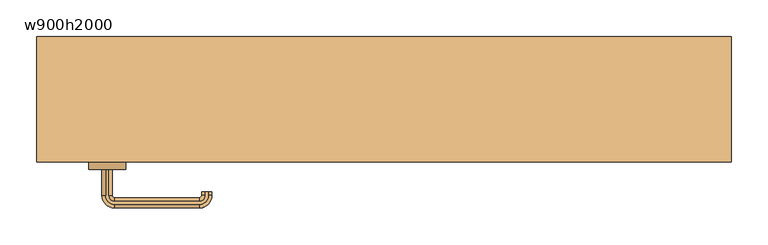
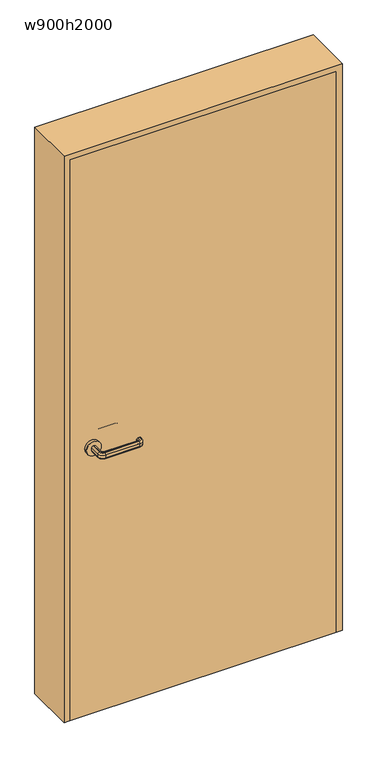
"""IFC4 building model written with IfcOpenShell, lengths in millimetres: door geometry, 片開き : w900h2000."""

from ifc_helpers import new_model, si_unit, point, frame, frame_2d, origin, origin_with_axes, place, context, project, spatial, polyline, circle_curve, ellipse_curve, trimmed, segment, composite_curve, outline, extrude, source, transform, mapped, element, save
from ifc_brep_helpers import plane_surface, cylinder_surface, revolved_surface, advanced_brep


def w900h2000_c063673d(model_context):
    return source(origin(), model_context, "Body", "SolidModel", [
        advanced_brep(
        [(-377.0, -95.0, 960.0), (-373.0, -95.0, 960.0), (-368.0, -95.0, 955.0), (-368.0, -95.0, 945.0477623), (-373.0, -95.0, 940.0477623), (-377.0, -95.0, 940.0477623), (-382.0, -95.0, 945.0477623), (-382.0, -95.0, 955.0), (-382.0, -130.0, 955.0), (-377.0, -130.0, 960.0), (-382.0, -130.0, 945.0477623), (-377.0, -130.0, 940.0477623), (-373.0, -130.0, 940.0477623), (-365.0, -138.0, 940.0477623), (-250.0, -138.0, 940.0477623), (-242.0, -130.0, 940.0477623), (-242.0, -125.0, 940.0477623), (-238.0, -125.0, 940.0477623), (-238.0, -130.0, 940.0477623), (-250.0, -142.0, 940.0477623), (-365.0, -142.0, 940.0477623), (-368.0, -130.0, 945.0477623), (-368.0, -130.0, 955.0), (-373.0, -130.0, 960.0), (-365.0, -142.0, 960.0), (-250.0, -142.0, 960.0), (-238.0, -130.0, 960.0), (-238.0, -125.0, 960.0), (-242.0, -125.0, 960.0), (-242.0, -130.0, 960.0), (-250.0, -138.0, 960.0), (-365.0, -138.0, 960.0), (-365.0, -147.0, 955.0), (-365.0, -147.0, 945.0477623), (-365.0, -133.0, 945.0477623), (-365.0, -133.0, 955.0), (-250.0, -147.0, 955.0), (-250.0, -147.0, 945.0477623), (-250.0, -133.0, 945.0477623), (-250.0, -133.0, 955.0), (-233.0, -130.0, 955.0), (-233.0, -130.0, 945.0477623), (-247.0, -130.0, 945.0477623), (-247.0, -130.0, 955.0), (-233.0, -125.0, 955.0), (-233.0, -125.0, 945.0477623), (-247.0, -125.0, 945.0477623), (-247.0, -125.0, 955.0)],
        [
            (0, 1),
            (1, 2, circle_curve(frame((-373.0, -95.0, 955.0), z_axis=(0.0, 1.0, 0.0), x_axis=(-1.0, 0.0, 0.0)), 5.0)),
            (2, 3),
            (3, 4, circle_curve(frame((-373.0, -95.0, 945.0477623), z_axis=(0.0, 1.0, 0.0), x_axis=(-1.0, 0.0, 0.0)), 5.0)),
            (4, 5),
            (5, 6, circle_curve(frame((-377.0, -95.0, 945.0477623), z_axis=(0.0, 1.0, 0.0), x_axis=(-1.0, 0.0, 0.0)), 5.0)),
            (6, 7),
            (7, 0, circle_curve(frame((-377.0, -95.0, 955.0), z_axis=(0.0, 1.0, 0.0), x_axis=(-1.0, 0.0, 0.0)), 5.0)),
            (7, 8),
            (8, 9, circle_curve(frame((-377.0, -130.0, 955.0), z_axis=(0.0, 1.0, 0.0), x_axis=(-1.0, 0.0, 0.0)), 5.0)),
            (9, 0),
            (6, 10),
            (10, 8),
            (5, 11),
            (11, 10, circle_curve(frame((-377.0, -130.0, 945.0477623), z_axis=(0.0, 1.0, 0.0), x_axis=(-1.0, 0.0, 0.0)), 5.0)),
            (4, 12),
            (12, 13, circle_curve(frame((-365.0, -130.0, 940.0477623), z_axis=(0.0, 0.0, 1.0), x_axis=(-1.0, 0.0, 0.0)), 8.0)),
            (13, 14),
            (14, 15, circle_curve(frame((-250.0, -130.0, 940.0477623), z_axis=(0.0, 0.0, 1.0), x_axis=(0.0, -1.0, 0.0)), 8.0)),
            (15, 16),
            (16, 17),
            (17, 18),
            (18, 19, circle_curve(frame((-250.0, -130.0, 940.0477623), z_axis=(0.0, 0.0, -1.0), x_axis=(0.0, -1.0, 0.0)), 12.0)),
            (19, 20),
            (20, 11, circle_curve(frame((-365.0, -130.0, 940.0477623), z_axis=(0.0, 0.0, -1.0), x_axis=(-1.0, 0.0, 0.0)), 12.0)),
            (3, 21),
            (21, 12, circle_curve(frame((-373.0, -130.0, 945.0477623), z_axis=(0.0, 1.0, 0.0), x_axis=(-1.0, 0.0, 0.0)), 5.0)),
            (2, 22),
            (22, 21),
            (1, 23),
            (23, 22, circle_curve(frame((-373.0, -130.0, 955.0), z_axis=(0.0, 1.0, 0.0), x_axis=(-1.0, 0.0, 0.0)), 5.0)),
            (9, 24, circle_curve(frame((-365.0, -130.0, 960.0), z_axis=(0.0, 0.0, 1.0), x_axis=(-1.0, 0.0, 0.0)), 12.0)),
            (24, 25),
            (25, 26, circle_curve(frame((-250.0, -130.0, 960.0), z_axis=(0.0, 0.0, 1.0), x_axis=(0.0, -1.0, 0.0)), 12.0)),
            (26, 27),
            (27, 28),
            (28, 29),
            (29, 30, circle_curve(frame((-250.0, -130.0, 960.0), z_axis=(0.0, 0.0, -1.0), x_axis=(0.0, -1.0, 0.0)), 8.0)),
            (30, 31),
            (31, 23, circle_curve(frame((-365.0, -130.0, 960.0), z_axis=(0.0, 0.0, -1.0), x_axis=(-1.0, 0.0, 0.0)), 8.0)),
            (32, 24, circle_curve(frame((-365.0, -142.0, 955.0), z_axis=(-1.0, 0.0, 0.0), x_axis=(0.0, -1.0, 0.0)), 5.0)),
            (8, 32, circle_curve(frame((-365.0, -130.0, 955.0), z_axis=(0.0, 0.0, 1.0), x_axis=(-1.0, 0.0, 0.0)), 17.0)),
            (33, 32),
            (10, 33, circle_curve(frame((-365.0, -130.0, 945.0477623), z_axis=(0.0, 0.0, 1.0), x_axis=(-1.0, 0.0, 0.0)), 17.0)),
            (20, 33, circle_curve(frame((-365.0, -142.0, 945.0477623), z_axis=(-1.0, 0.0, 0.0), x_axis=(0.0, -1.0, 0.0)), 5.0)),
            (34, 13, circle_curve(frame((-365.0, -138.0, 945.0477623), z_axis=(-1.0, 0.0, 0.0), x_axis=(0.0, -1.0, 0.0)), 5.0)),
            (21, 34, circle_curve(frame((-365.0, -130.0, 945.0477623), z_axis=(0.0, 0.0, 1.0), x_axis=(-1.0, 0.0, 0.0)), 3.0)),
            (35, 34),
            (22, 35, circle_curve(frame((-365.0, -130.0, 955.0), z_axis=(0.0, 0.0, 1.0), x_axis=(-1.0, 0.0, 0.0)), 3.0)),
            (31, 35, circle_curve(frame((-365.0, -138.0, 955.0), z_axis=(-1.0, 0.0, 0.0), x_axis=(0.0, -1.0, 0.0)), 5.0)),
            (32, 36),
            (36, 25, circle_curve(frame((-250.0, -142.0, 955.0), z_axis=(-1.0, 0.0, 0.0), x_axis=(0.0, -1.0, 0.0)), 5.0)),
            (33, 37),
            (37, 36),
            (19, 37, circle_curve(frame((-250.0, -142.0, 945.0477623), z_axis=(-1.0, 0.0, 0.0), x_axis=(0.0, -1.0, 0.0)), 5.0)),
            (34, 38),
            (38, 14, circle_curve(frame((-250.0, -138.0, 945.0477623), z_axis=(-1.0, 0.0, 0.0), x_axis=(0.0, -1.0, 0.0)), 5.0)),
            (35, 39),
            (39, 38),
            (30, 39, circle_curve(frame((-250.0, -138.0, 955.0), z_axis=(-1.0, 0.0, 0.0), x_axis=(0.0, -1.0, 0.0)), 5.0)),
            (40, 26, circle_curve(frame((-238.0, -130.0, 955.0), z_axis=(0.0, -1.0, 0.0), x_axis=(1.0, 0.0, 0.0)), 5.0)),
            (36, 40, circle_curve(frame((-250.0, -130.0, 955.0), z_axis=(0.0, 0.0, 1.0), x_axis=(0.0, -1.0, 0.0)), 17.0)),
            (41, 40),
            (37, 41, circle_curve(frame((-250.0, -130.0, 945.0477623), z_axis=(0.0, 0.0, 1.0), x_axis=(0.0, -1.0, 0.0)), 17.0)),
            (18, 41, circle_curve(frame((-238.0, -130.0, 945.0477623), z_axis=(0.0, -1.0, 0.0), x_axis=(1.0, 0.0, 0.0)), 5.0)),
            (42, 15, circle_curve(frame((-242.0, -130.0, 945.0477623), z_axis=(0.0, -1.0, 0.0), x_axis=(1.0, 0.0, 0.0)), 5.0)),
            (38, 42, circle_curve(frame((-250.0, -130.0, 945.0477623), z_axis=(0.0, 0.0, 1.0), x_axis=(0.0, -1.0, 0.0)), 3.0)),
            (43, 42),
            (39, 43, circle_curve(frame((-250.0, -130.0, 955.0), z_axis=(0.0, 0.0, 1.0), x_axis=(0.0, -1.0, 0.0)), 3.0)),
            (29, 43, circle_curve(frame((-242.0, -130.0, 955.0), z_axis=(0.0, -1.0, 0.0), x_axis=(1.0, 0.0, 0.0)), 5.0)),
            (27, 44, circle_curve(frame((-238.0, -125.0, 955.0), z_axis=(0.0, 1.0, 0.0), x_axis=(1.0, 0.0, 0.0)), 5.0)),
            (44, 45),
            (45, 17, circle_curve(frame((-238.0, -125.0, 945.0477623), z_axis=(0.0, 1.0, 0.0), x_axis=(1.0, 0.0, 0.0)), 5.0)),
            (16, 46, circle_curve(frame((-242.0, -125.0, 945.0477623), z_axis=(0.0, 1.0, 0.0), x_axis=(1.0, 0.0, 0.0)), 5.0)),
            (46, 47),
            (47, 28, circle_curve(frame((-242.0, -125.0, 955.0), z_axis=(0.0, 1.0, 0.0), x_axis=(1.0, 0.0, 0.0)), 5.0)),
            (40, 44),
            (41, 45),
            (42, 46),
            (43, 47),
        ],
        [
            plane_surface(frame((-385.198039, -95.0, 950.0), z_axis=(0.0, 1.0, 0.0), x_axis=(0.0, 0.0, 1.0))),
            cylinder_surface(frame((-377.0, -95.0, 955.0), z_axis=(0.0, 1.0, 0.0), x_axis=(-1.0, 0.0, 0.0)), 5.0),
            plane_surface(frame((-382.0, -95.0, 955.0), z_axis=(-1.0, 0.0, 0.0), x_axis=(0.0, -1.0, 0.0))),
            cylinder_surface(frame((-377.0, -95.0, 945.0477623), z_axis=(0.0, 1.0, 0.0), x_axis=(-1.0, 0.0, 0.0)), 5.0),
            plane_surface(frame((-377.0, -95.0, 940.0477623), z_axis=(0.0, 0.0, -1.0), x_axis=(0.0, -1.0, 0.0))),
            cylinder_surface(frame((-373.0, -95.0, 945.0477623), z_axis=(0.0, 1.0, 0.0), x_axis=(-1.0, 0.0, 0.0)), 5.0),
            plane_surface(frame((-368.0, -95.0, 945.0477623), z_axis=(1.0, 0.0, 0.0), x_axis=(0.0, -1.0, 0.0))),
            cylinder_surface(frame((-373.0, -95.0, 955.0), z_axis=(0.0, 1.0, 0.0), x_axis=(-1.0, 0.0, 0.0)), 5.0),
            plane_surface(frame((-373.0, -95.0, 960.0), z_axis=(0.0, 0.0, 1.0), x_axis=(0.0, -1.0, 0.0))),
            revolved_surface(trimmed(ellipse_curve(frame((-377.0, -130.0, 955.0), z_axis=(0.0, -1.0, 0.0), x_axis=(-1.0, 0.0, 0.0)), 5.0, 5.0), [point((-377.0, -130.0, 960.0))], [point((-382.0, -130.0, 955.0))], True, "CARTESIAN"), (-365.0, -130.0, 950.0), (0.0, 0.0, -1.0)),
            cylinder_surface(frame((-365.0, -130.0, 950.0), z_axis=(0.0, 0.0, -1.0), x_axis=(-1.0, 0.0, 0.0)), 17.0),
            revolved_surface(trimmed(ellipse_curve(frame((-377.0, -130.0, 945.0477623), z_axis=(0.0, -1.0, 0.0), x_axis=(-1.0, 0.0, 0.0)), 5.0, 5.0), [point((-382.0, -130.0, 945.0477623))], [point((-377.0, -130.0, 940.0477623))], True, "CARTESIAN"), (-365.0, -130.0, 950.0), (0.0, 0.0, -1.0)),
            revolved_surface(trimmed(ellipse_curve(frame((-373.0, -130.0, 945.0477623), z_axis=(0.0, -1.0, 0.0), x_axis=(-1.0, 0.0, 0.0)), 5.0, 5.0), [point((-373.0, -130.0, 940.0477623))], [point((-368.0, -130.0, 945.0477623))], True, "CARTESIAN"), (-365.0, -130.0, 950.0), (0.0, 0.0, -1.0)),
            revolved_surface(polyline([(-368.0, -130.0, 945.0477623), (-368.0, -130.0, 955.0)]), (-365.0, -130.0, 950.0), (0.0, 0.0, -1.0)),
            revolved_surface(trimmed(ellipse_curve(frame((-373.0, -130.0, 955.0), z_axis=(0.0, -1.0, 0.0), x_axis=(-1.0, 0.0, 0.0)), 5.0, 5.0), [point((-368.0, -130.0, 955.0))], [point((-373.0, -130.0, 960.0))], True, "CARTESIAN"), (-365.0, -130.0, 950.0), (0.0, 0.0, -1.0)),
            cylinder_surface(frame((-365.0, -142.0, 955.0), z_axis=(-1.0, 0.0, 0.0), x_axis=(0.0, -1.0, 0.0)), 5.0),
            plane_surface(frame((-365.0, -147.0, 955.0), z_axis=(0.0, -1.0, 0.0), x_axis=(1.0, 0.0, 0.0))),
            cylinder_surface(frame((-365.0, -142.0, 945.0477623), z_axis=(-1.0, 0.0, 0.0), x_axis=(0.0, -1.0, 0.0)), 5.0),
            cylinder_surface(frame((-365.0, -138.0, 945.0477623), z_axis=(-1.0, 0.0, 0.0), x_axis=(0.0, -1.0, 0.0)), 5.0),
            plane_surface(frame((-365.0, -133.0, 945.0477623), z_axis=(0.0, 1.0, 0.0), x_axis=(1.0, 0.0, 0.0))),
            cylinder_surface(frame((-365.0, -138.0, 955.0), z_axis=(-1.0, 0.0, 0.0), x_axis=(0.0, -1.0, 0.0)), 5.0),
            revolved_surface(trimmed(ellipse_curve(frame((-250.0, -142.0, 955.0), z_axis=(1.0, 0.0, 0.0), x_axis=(0.0, -1.0, 0.0)), 5.0, 5.0), [point((-250.0, -142.0, 960.0))], [point((-250.0, -147.0, 955.0))], True, "CARTESIAN"), (-250.0, -130.0, 950.0), (0.0, 0.0, -1.0)),
            cylinder_surface(frame((-250.0, -130.0, 950.0), z_axis=(0.0, 0.0, -1.0), x_axis=(0.0, -1.0, 0.0)), 17.0),
            revolved_surface(trimmed(ellipse_curve(frame((-250.0, -142.0, 945.0477623), z_axis=(1.0, 0.0, 0.0), x_axis=(0.0, -1.0, 0.0)), 5.0, 5.0), [point((-250.0, -147.0, 945.0477623))], [point((-250.0, -142.0, 940.0477623))], True, "CARTESIAN"), (-250.0, -130.0, 950.0), (0.0, 0.0, -1.0)),
            revolved_surface(trimmed(ellipse_curve(frame((-250.0, -138.0, 945.0477623), z_axis=(1.0, 0.0, 0.0), x_axis=(0.0, -1.0, 0.0)), 5.0, 5.0), [point((-250.0, -138.0, 940.0477623))], [point((-250.0, -133.0, 945.0477623))], True, "CARTESIAN"), (-250.0, -130.0, 950.0), (0.0, 0.0, -1.0)),
            revolved_surface(polyline([(-250.0, -133.0, 945.0477623), (-250.0, -133.0, 955.0)]), (-250.0, -130.0, 950.0), (0.0, 0.0, -1.0)),
            revolved_surface(trimmed(ellipse_curve(frame((-250.0, -138.0, 955.0), z_axis=(1.0, 0.0, 0.0), x_axis=(0.0, -1.0, 0.0)), 5.0, 5.0), [point((-250.0, -133.0, 955.0))], [point((-250.0, -138.0, 960.0))], True, "CARTESIAN"), (-250.0, -130.0, 950.0), (0.0, 0.0, -1.0)),
            plane_surface(frame((-250.198039, -125.0, 950.0), z_axis=(0.0, 1.0, 0.0), x_axis=(0.0, 0.0, -1.0))),
            cylinder_surface(frame((-238.0, -130.0, 955.0), z_axis=(0.0, -1.0, 0.0), x_axis=(1.0, 0.0, 0.0)), 5.0),
            plane_surface(frame((-233.0, -130.0, 955.0), z_axis=(1.0, 0.0, 0.0), x_axis=(0.0, 1.0, 0.0))),
            cylinder_surface(frame((-238.0, -130.0, 945.0477623), z_axis=(0.0, -1.0, 0.0), x_axis=(1.0, 0.0, 0.0)), 5.0),
            cylinder_surface(frame((-242.0, -130.0, 945.0477623), z_axis=(0.0, -1.0, 0.0), x_axis=(1.0, 0.0, 0.0)), 5.0),
            plane_surface(frame((-247.0, -130.0, 945.0477623), z_axis=(-1.0, 0.0, 0.0), x_axis=(0.0, 1.0, 0.0))),
            cylinder_surface(frame((-242.0, -130.0, 955.0), z_axis=(0.0, -1.0, 0.0), x_axis=(1.0, 0.0, 0.0)), 5.0),
        ],
        [
            (0, [[1, 2, 3, 4, 5, 6, 7, 8]]),
            (1, [[9, 10, 11, -8]]),
            (2, [[12, 13, -9, -7]]),
            (3, [[14, 15, -12, -6]]),
            (4, [[16, 17, 18, 19, 20, 21, 22, 23, 24, 25, -14, -5]]),
            (5, [[26, 27, -16, -4]]),
            (6, [[28, 29, -26, -3]]),
            (7, [[30, 31, -28, -2]]),
            (8, [[-11, 32, 33, 34, 35, 36, 37, 38, 39, 40, -30, -1]]),
            (9, [[41, -32, -10, 42]]),
            (10, [[43, -42, -13, 44]]),
            (11, [[45, -44, -15, -25]]),
            (12, [[46, -17, -27, 47]]),
            (13, [[48, -47, -29, 49]]),
            (14, [[50, -49, -31, -40]]),
            (15, [[51, 52, -33, -41]]),
            (16, [[53, 54, -51, -43]]),
            (17, [[-24, 55, -53, -45]]),
            (18, [[56, 57, -18, -46]]),
            (19, [[58, 59, -56, -48]]),
            (20, [[-39, 60, -58, -50]]),
            (21, [[61, -34, -52, 62]]),
            (22, [[63, -62, -54, 64]]),
            (23, [[65, -64, -55, -23]]),
            (24, [[66, -19, -57, 67]]),
            (25, [[68, -67, -59, 69]]),
            (26, [[70, -69, -60, -38]]),
            (27, [[71, 72, 73, -21, 74, 75, 76, -36]]),
            (28, [[77, -71, -35, -61]]),
            (29, [[78, -72, -77, -63]]),
            (30, [[-22, -73, -78, -65]]),
            (31, [[79, -74, -20, -66]]),
            (32, [[80, -75, -79, -68]]),
            (33, [[-37, -76, -80, -70]]),
        ],
    ),
        advanced_brep(
        [(-373.0, -45.0, 940.0), (-368.0, -45.0, 945.0), (-368.0, -45.0, 955.0), (-373.0, -45.0, 960.0), (-377.0, -45.0, 960.0), (-382.0, -45.0, 955.0), (-382.0, -45.0, 945.0), (-377.0, -45.0, 940.0), (-377.0, -10.0, 940.0), (-365.0, 2.0, 940.0), (-250.0, 2.0, 940.0), (-238.0, -10.0, 940.0), (-238.0, -15.0, 940.0), (-242.0, -15.0, 940.0), (-242.0, -10.0, 940.0), (-250.0, -2.0, 940.0), (-365.0, -2.0, 940.0), (-373.0, -10.0, 940.0), (-382.0, -10.0, 945.0), (-382.0, -10.0, 955.0), (-377.0, -10.0, 960.0), (-373.0, -10.0, 960.0), (-365.0, -2.0, 960.0), (-250.0, -2.0, 960.0), (-242.0, -10.0, 960.0), (-242.0, -15.0, 960.0), (-238.0, -15.0, 960.0), (-238.0, -10.0, 960.0), (-250.0, 2.0, 960.0), (-365.0, 2.0, 960.0), (-368.0, -10.0, 955.0), (-368.0, -10.0, 945.0), (-365.0, 7.0, 945.0), (-365.0, 7.0, 955.0), (-365.0, -7.0, 955.0), (-365.0, -7.0, 945.0), (-250.0, 7.0, 945.0), (-250.0, 7.0, 955.0), (-250.0, -7.0, 955.0), (-250.0, -7.0, 945.0), (-233.0, -10.0, 945.0), (-233.0, -10.0, 955.0), (-247.0, -10.0, 955.0), (-247.0, -10.0, 945.0), (-233.0, -15.0, 945.0), (-233.0, -15.0, 955.0), (-247.0, -15.0, 955.0), (-247.0, -15.0, 945.0)],
        [
            (0, 1, circle_curve(frame((-373.0, -45.0, 945.0), z_axis=(0.0, -1.0, 0.0), x_axis=(1.0, 0.0, 0.0)), 5.0)),
            (1, 2),
            (2, 3, circle_curve(frame((-373.0, -45.0, 955.0), z_axis=(0.0, -1.0, 0.0), x_axis=(1.0, 0.0, 0.0)), 5.0)),
            (3, 4),
            (4, 5, circle_curve(frame((-377.0, -45.0, 955.0), z_axis=(0.0, -1.0, 0.0), x_axis=(1.0, 0.0, 0.0)), 5.0)),
            (5, 6),
            (6, 7, circle_curve(frame((-377.0, -45.0, 945.0), z_axis=(0.0, -1.0, 0.0), x_axis=(1.0, 0.0, 0.0)), 5.0)),
            (7, 0),
            (7, 8),
            (8, 9, circle_curve(frame((-365.0, -10.0, 940.0), z_axis=(0.0, 0.0, -1.0), x_axis=(-1.0, 0.0, 0.0)), 12.0)),
            (9, 10),
            (10, 11, circle_curve(frame((-250.0, -10.0, 940.0), z_axis=(0.0, 0.0, -1.0), x_axis=(0.0, 1.0, 0.0)), 12.0)),
            (11, 12),
            (12, 13),
            (13, 14),
            (14, 15, circle_curve(frame((-250.0, -10.0, 940.0), z_axis=(0.0, 0.0, 1.0), x_axis=(0.0, 1.0, 0.0)), 8.0)),
            (15, 16),
            (16, 17, circle_curve(frame((-365.0, -10.0, 940.0), z_axis=(0.0, 0.0, 1.0), x_axis=(-1.0, 0.0, 0.0)), 8.0)),
            (17, 0),
            (6, 18),
            (18, 8, circle_curve(frame((-377.0, -10.0, 945.0), z_axis=(0.0, -1.0, 0.0), x_axis=(1.0, 0.0, 0.0)), 5.0)),
            (5, 19),
            (19, 18),
            (4, 20),
            (20, 19, circle_curve(frame((-377.0, -10.0, 955.0), z_axis=(0.0, -1.0, 0.0), x_axis=(1.0, 0.0, 0.0)), 5.0)),
            (3, 21),
            (21, 22, circle_curve(frame((-365.0, -10.0, 960.0), z_axis=(0.0, 0.0, -1.0), x_axis=(-1.0, 0.0, 0.0)), 8.0)),
            (22, 23),
            (23, 24, circle_curve(frame((-250.0, -10.0, 960.0), z_axis=(0.0, 0.0, -1.0), x_axis=(0.0, 1.0, 0.0)), 8.0)),
            (24, 25),
            (25, 26),
            (26, 27),
            (27, 28, circle_curve(frame((-250.0, -10.0, 960.0), z_axis=(0.0, 0.0, 1.0), x_axis=(0.0, 1.0, 0.0)), 12.0)),
            (28, 29),
            (29, 20, circle_curve(frame((-365.0, -10.0, 960.0), z_axis=(0.0, 0.0, 1.0), x_axis=(-1.0, 0.0, 0.0)), 12.0)),
            (2, 30),
            (30, 21, circle_curve(frame((-373.0, -10.0, 955.0), z_axis=(0.0, -1.0, 0.0), x_axis=(1.0, 0.0, 0.0)), 5.0)),
            (1, 31),
            (31, 30),
            (17, 31, circle_curve(frame((-373.0, -10.0, 945.0), z_axis=(0.0, -1.0, 0.0), x_axis=(1.0, 0.0, 0.0)), 5.0)),
            (32, 9, circle_curve(frame((-365.0, 2.0, 945.0), z_axis=(-1.0, 0.0, 0.0), x_axis=(0.0, -1.0, 0.0)), 5.0)),
            (18, 32, circle_curve(frame((-365.0, -10.0, 945.0), z_axis=(0.0, 0.0, -1.0), x_axis=(-1.0, 0.0, 0.0)), 17.0)),
            (33, 32),
            (19, 33, circle_curve(frame((-365.0, -10.0, 955.0), z_axis=(0.0, 0.0, -1.0), x_axis=(-1.0, 0.0, 0.0)), 17.0)),
            (29, 33, circle_curve(frame((-365.0, 2.0, 955.0), z_axis=(-1.0, 0.0, 0.0), x_axis=(0.0, -1.0, 0.0)), 5.0)),
            (34, 22, circle_curve(frame((-365.0, -2.0, 955.0), z_axis=(-1.0, 0.0, 0.0), x_axis=(0.0, -1.0, 0.0)), 5.0)),
            (30, 34, circle_curve(frame((-365.0, -10.0, 955.0), z_axis=(0.0, 0.0, -1.0), x_axis=(-1.0, 0.0, 0.0)), 3.0)),
            (35, 34),
            (31, 35, circle_curve(frame((-365.0, -10.0, 945.0), z_axis=(0.0, 0.0, -1.0), x_axis=(-1.0, 0.0, 0.0)), 3.0)),
            (16, 35, circle_curve(frame((-365.0, -2.0, 945.0), z_axis=(-1.0, 0.0, 0.0), x_axis=(0.0, -1.0, 0.0)), 5.0)),
            (32, 36),
            (36, 10, circle_curve(frame((-250.0, 2.0, 945.0), z_axis=(-1.0, 0.0, 0.0), x_axis=(0.0, -1.0, 0.0)), 5.0)),
            (33, 37),
            (37, 36),
            (28, 37, circle_curve(frame((-250.0, 2.0, 955.0), z_axis=(-1.0, 0.0, 0.0), x_axis=(0.0, -1.0, 0.0)), 5.0)),
            (34, 38),
            (38, 23, circle_curve(frame((-250.0, -2.0, 955.0), z_axis=(-1.0, 0.0, 0.0), x_axis=(0.0, -1.0, 0.0)), 5.0)),
            (35, 39),
            (39, 38),
            (15, 39, circle_curve(frame((-250.0, -2.0, 945.0), z_axis=(-1.0, 0.0, 0.0), x_axis=(0.0, -1.0, 0.0)), 5.0)),
            (40, 11, circle_curve(frame((-238.0, -10.0, 945.0), z_axis=(0.0, 1.0, 0.0), x_axis=(-1.0, 0.0, 0.0)), 5.0)),
            (36, 40, circle_curve(frame((-250.0, -10.0, 945.0), z_axis=(0.0, 0.0, -1.0), x_axis=(0.0, 1.0, 0.0)), 17.0)),
            (41, 40),
            (37, 41, circle_curve(frame((-250.0, -10.0, 955.0), z_axis=(0.0, 0.0, -1.0), x_axis=(0.0, 1.0, 0.0)), 17.0)),
            (27, 41, circle_curve(frame((-238.0, -10.0, 955.0), z_axis=(0.0, 1.0, 0.0), x_axis=(-1.0, 0.0, 0.0)), 5.0)),
            (42, 24, circle_curve(frame((-242.0, -10.0, 955.0), z_axis=(0.0, 1.0, 0.0), x_axis=(-1.0, 0.0, 0.0)), 5.0)),
            (38, 42, circle_curve(frame((-250.0, -10.0, 955.0), z_axis=(0.0, 0.0, -1.0), x_axis=(0.0, 1.0, 0.0)), 3.0)),
            (43, 42),
            (39, 43, circle_curve(frame((-250.0, -10.0, 945.0), z_axis=(0.0, 0.0, -1.0), x_axis=(0.0, 1.0, 0.0)), 3.0)),
            (14, 43, circle_curve(frame((-242.0, -10.0, 945.0), z_axis=(0.0, 1.0, 0.0), x_axis=(-1.0, 0.0, 0.0)), 5.0)),
            (12, 44, circle_curve(frame((-238.0, -15.0, 945.0), z_axis=(0.0, -1.0, 0.0), x_axis=(-1.0, 0.0, 0.0)), 5.0)),
            (44, 45),
            (45, 26, circle_curve(frame((-238.0, -15.0, 955.0), z_axis=(0.0, -1.0, 0.0), x_axis=(-1.0, 0.0, 0.0)), 5.0)),
            (25, 46, circle_curve(frame((-242.0, -15.0, 955.0), z_axis=(0.0, -1.0, 0.0), x_axis=(-1.0, 0.0, 0.0)), 5.0)),
            (46, 47),
            (47, 13, circle_curve(frame((-242.0, -15.0, 945.0), z_axis=(0.0, -1.0, 0.0), x_axis=(-1.0, 0.0, 0.0)), 5.0)),
            (40, 44),
            (41, 45),
            (42, 46),
            (43, 47),
        ],
        [
            plane_surface(frame((-385.198039, -45.0, 950.0), z_axis=(0.0, -1.0, 0.0), x_axis=(0.0, 0.0, -1.0))),
            plane_surface(frame((-373.0, -45.0, 940.0), z_axis=(0.0, 0.0, -1.0), x_axis=(0.0, 1.0, 0.0))),
            cylinder_surface(frame((-377.0, -45.0, 945.0), z_axis=(0.0, -1.0, 0.0), x_axis=(1.0, 0.0, 0.0)), 5.0),
            plane_surface(frame((-382.0, -45.0, 945.0), z_axis=(-1.0, 0.0, 0.0), x_axis=(0.0, 1.0, 0.0))),
            cylinder_surface(frame((-377.0, -45.0, 955.0), z_axis=(0.0, -1.0, 0.0), x_axis=(1.0, 0.0, 0.0)), 5.0),
            plane_surface(frame((-377.0, -45.0, 960.0), z_axis=(0.0, 0.0, 1.0), x_axis=(0.0, 1.0, 0.0))),
            cylinder_surface(frame((-373.0, -45.0, 955.0), z_axis=(0.0, -1.0, 0.0), x_axis=(1.0, 0.0, 0.0)), 5.0),
            plane_surface(frame((-368.0, -45.0, 955.0), z_axis=(1.0, 0.0, 0.0), x_axis=(0.0, 1.0, 0.0))),
            cylinder_surface(frame((-373.0, -45.0, 945.0), z_axis=(0.0, -1.0, 0.0), x_axis=(1.0, 0.0, 0.0)), 5.0),
            revolved_surface(trimmed(ellipse_curve(frame((-377.0, -10.0, 945.0), z_axis=(0.0, 1.0, 0.0), x_axis=(1.0, 0.0, 0.0)), 5.0, 5.0), [point((-377.0, -10.0, 940.0))], [point((-382.0, -10.0, 945.0))], True, "CARTESIAN"), (-365.0, -10.0, 950.0), (0.0, 0.0, 1.0)),
            cylinder_surface(frame((-365.0, -10.0, 950.0), z_axis=(0.0, 0.0, 1.0), x_axis=(-1.0, 0.0, 0.0)), 17.0),
            revolved_surface(trimmed(ellipse_curve(frame((-377.0, -10.0, 955.0), z_axis=(0.0, 1.0, 0.0), x_axis=(1.0, 0.0, 0.0)), 5.0, 5.0), [point((-382.0, -10.0, 955.0))], [point((-377.0, -10.0, 960.0))], True, "CARTESIAN"), (-365.0, -10.0, 950.0), (0.0, 0.0, 1.0)),
            revolved_surface(trimmed(ellipse_curve(frame((-373.0, -10.0, 955.0), z_axis=(0.0, 1.0, 0.0), x_axis=(1.0, 0.0, 0.0)), 5.0, 5.0), [point((-373.0, -10.0, 960.0))], [point((-368.0, -10.0, 955.0))], True, "CARTESIAN"), (-365.0, -10.0, 950.0), (0.0, 0.0, 1.0)),
            revolved_surface(polyline([(-368.0, -10.0, 955.0), (-368.0, -10.0, 945.0)]), (-365.0, -10.0, 950.0), (0.0, 0.0, 1.0)),
            revolved_surface(trimmed(ellipse_curve(frame((-373.0, -10.0, 945.0), z_axis=(0.0, 1.0, 0.0), x_axis=(1.0, 0.0, 0.0)), 5.0, 5.0), [point((-368.0, -10.0, 945.0))], [point((-373.0, -10.0, 940.0))], True, "CARTESIAN"), (-365.0, -10.0, 950.0), (0.0, 0.0, 1.0)),
            cylinder_surface(frame((-365.0, 2.0, 945.0), z_axis=(-1.0, 0.0, 0.0), x_axis=(0.0, -1.0, 0.0)), 5.0),
            plane_surface(frame((-365.0, 7.0, 945.0), z_axis=(0.0, 1.0, 0.0), x_axis=(1.0, 0.0, 0.0))),
            cylinder_surface(frame((-365.0, 2.0, 955.0), z_axis=(-1.0, 0.0, 0.0), x_axis=(0.0, -1.0, 0.0)), 5.0),
            cylinder_surface(frame((-365.0, -2.0, 955.0), z_axis=(-1.0, 0.0, 0.0), x_axis=(0.0, -1.0, 0.0)), 5.0),
            plane_surface(frame((-365.0, -7.0, 955.0), z_axis=(0.0, -1.0, 0.0), x_axis=(1.0, 0.0, 0.0))),
            cylinder_surface(frame((-365.0, -2.0, 945.0), z_axis=(-1.0, 0.0, 0.0), x_axis=(0.0, -1.0, 0.0)), 5.0),
            revolved_surface(trimmed(ellipse_curve(frame((-250.0, 2.0, 945.0), z_axis=(1.0, 0.0, 0.0), x_axis=(0.0, -1.0, 0.0)), 5.0, 5.0), [point((-250.0, 2.0, 940.0))], [point((-250.0, 7.0, 945.0))], True, "CARTESIAN"), (-250.0, -10.0, 950.0), (0.0, 0.0, 1.0)),
            cylinder_surface(frame((-250.0, -10.0, 950.0), z_axis=(0.0, 0.0, 1.0), x_axis=(0.0, 1.0, 0.0)), 17.0),
            revolved_surface(trimmed(ellipse_curve(frame((-250.0, 2.0, 955.0), z_axis=(1.0, 0.0, 0.0), x_axis=(0.0, -1.0, 0.0)), 5.0, 5.0), [point((-250.0, 7.0, 955.0))], [point((-250.0, 2.0, 960.0))], True, "CARTESIAN"), (-250.0, -10.0, 950.0), (0.0, 0.0, 1.0)),
            revolved_surface(trimmed(ellipse_curve(frame((-250.0, -2.0, 955.0), z_axis=(1.0, 0.0, 0.0), x_axis=(0.0, -1.0, 0.0)), 5.0, 5.0), [point((-250.0, -2.0, 960.0))], [point((-250.0, -7.0, 955.0))], True, "CARTESIAN"), (-250.0, -10.0, 950.0), (0.0, 0.0, 1.0)),
            revolved_surface(polyline([(-250.0, -7.0, 955.0), (-250.0, -7.0, 945.0)]), (-250.0, -10.0, 950.0), (0.0, 0.0, 1.0)),
            revolved_surface(trimmed(ellipse_curve(frame((-250.0, -2.0, 945.0), z_axis=(1.0, 0.0, 0.0), x_axis=(0.0, -1.0, 0.0)), 5.0, 5.0), [point((-250.0, -7.0, 945.0))], [point((-250.0, -2.0, 940.0))], True, "CARTESIAN"), (-250.0, -10.0, 950.0), (0.0, 0.0, 1.0)),
            plane_surface(frame((-250.198039, -15.0, 950.0), z_axis=(0.0, -1.0, 0.0), x_axis=(0.0, 0.0, 1.0))),
            cylinder_surface(frame((-238.0, -10.0, 945.0), z_axis=(0.0, 1.0, 0.0), x_axis=(-1.0, 0.0, 0.0)), 5.0),
            plane_surface(frame((-233.0, -10.0, 945.0), z_axis=(1.0, 0.0, 0.0), x_axis=(0.0, -1.0, 0.0))),
            cylinder_surface(frame((-238.0, -10.0, 955.0), z_axis=(0.0, 1.0, 0.0), x_axis=(-1.0, 0.0, 0.0)), 5.0),
            cylinder_surface(frame((-242.0, -10.0, 955.0), z_axis=(0.0, 1.0, 0.0), x_axis=(-1.0, 0.0, 0.0)), 5.0),
            plane_surface(frame((-247.0, -10.0, 955.0), z_axis=(-1.0, 0.0, 0.0), x_axis=(0.0, -1.0, 0.0))),
            cylinder_surface(frame((-242.0, -10.0, 945.0), z_axis=(0.0, 1.0, 0.0), x_axis=(-1.0, 0.0, 0.0)), 5.0),
        ],
        [
            (0, [[1, 2, 3, 4, 5, 6, 7, 8]]),
            (1, [[9, 10, 11, 12, 13, 14, 15, 16, 17, 18, 19, -8]]),
            (2, [[20, 21, -9, -7]]),
            (3, [[22, 23, -20, -6]]),
            (4, [[24, 25, -22, -5]]),
            (5, [[26, 27, 28, 29, 30, 31, 32, 33, 34, 35, -24, -4]]),
            (6, [[36, 37, -26, -3]]),
            (7, [[38, 39, -36, -2]]),
            (8, [[-19, 40, -38, -1]]),
            (9, [[41, -10, -21, 42]]),
            (10, [[43, -42, -23, 44]]),
            (11, [[45, -44, -25, -35]]),
            (12, [[46, -27, -37, 47]]),
            (13, [[48, -47, -39, 49]]),
            (14, [[50, -49, -40, -18]]),
            (15, [[51, 52, -11, -41]]),
            (16, [[53, 54, -51, -43]]),
            (17, [[-34, 55, -53, -45]]),
            (18, [[56, 57, -28, -46]]),
            (19, [[58, 59, -56, -48]]),
            (20, [[-17, 60, -58, -50]]),
            (21, [[61, -12, -52, 62]]),
            (22, [[63, -62, -54, 64]]),
            (23, [[65, -64, -55, -33]]),
            (24, [[66, -29, -57, 67]]),
            (25, [[68, -67, -59, 69]]),
            (26, [[70, -69, -60, -16]]),
            (27, [[-14, 71, 72, 73, -31, 74, 75, 76]]),
            (28, [[77, -71, -13, -61]]),
            (29, [[78, -72, -77, -63]]),
            (30, [[-32, -73, -78, -65]]),
            (31, [[79, -74, -30, -66]]),
            (32, [[80, -75, -79, -68]]),
            (33, [[-15, -76, -80, -70]]),
        ],
    ),
        extrude(outline(composite_curve([segment(trimmed(circle_curve(frame_2d((950.0, -375.0)), 25.0), [point((950.0, -400.0))], [point((950.0, -350.0))], False, "CARTESIAN"), True, "CONTINUOUS"), segment(trimmed(circle_curve(frame_2d((950.0, -375.0)), 25.0), [point((950.0, -350.0))], [point((950.0, -400.0))], False, "CARTESIAN"), True, "CONTINUOUS")], self_intersect=False)), frame((0.0, -95.0, 0.0), z_axis=(0.0, 1.0, 0.0), x_axis=(0.0, 0.0, 1.0)), (0.0, 0.0, 1.0), 10.0),
        extrude(outline(composite_curve([segment(trimmed(circle_curve(frame_2d((950.0, -375.0)), 25.0), [point((950.0, -400.0))], [point((950.0, -350.0))], False, "CARTESIAN"), True, "CONTINUOUS"), segment(trimmed(circle_curve(frame_2d((950.0, -375.0)), 25.0), [point((950.0, -350.0))], [point((950.0, -400.0))], False, "CARTESIAN"), True, "CONTINUOUS")], self_intersect=False)), frame((0.0, -55.0, 0.0), z_axis=(0.0, 1.0, 0.0), x_axis=(0.0, 0.0, 1.0)), (0.0, 0.0, 1.0), 10.0),
        extrude(outline(polyline([(2020.0, -470.0), (0.0, -470.0), (0.0, -450.0), (2000.0, -450.0), (2000.0, 450.0), (0.0, 450.0), (0.0, 470.0), (2020.0, 470.0), (2020.0, -470.0)])), frame((0.0, -85.0, 0.0), z_axis=(0.0, 1.0, 0.0), x_axis=(0.0, 0.0, 1.0)), (0.0, 0.0, 1.0), 170.0),
        extrude(outline(polyline([(450.0, -55.0), (450.0, -85.0), (-450.0, -85.0), (-450.0, -55.0), (450.0, -55.0)])), origin_with_axes(), (0.0, 0.0, 1.0), 2000.0),
    ])


if __name__ == "__main__":
    model = new_model("IFC4")
    model_context = context("Model", 3, world=origin())
    ifc_project = project(units=[si_unit("LENGTHUNIT", "METRE", prefix="MILLI")], contexts=[model_context])
    site = spatial("IfcSite", under=ifc_project)
    building = spatial("IfcBuilding", under=site)
    placement = place(None, origin())
    w900h2000_shape = w900h2000_c063673d(model_context)
    element("IfcDoor", 1, ObjectType="片開き : w900h2000", at=placement, inside=building, context=model_context, shape_type="MappedRepresentation", body=[
        mapped(w900h2000_shape, transform((0.0, 0.0, 0.0), x_axis=(1.0, 0.0, 0.0), y_axis=(0.0, 1.0, 0.0), z_axis=(0.0, 0.0, 1.0))),
    ])
    save(model, "model.ifc")

# Revit data of these elements
# Project information
#   プロジェクト発行日 = "発行日"
#   プロジェクト ステータス = "プロジェクト ステータス"
#   クライアント名 = "オーナ"
#   計画地住所 = "ここにアドレスを入力"
#   プロジェクト名 = "プロジェクト名"
#   プロジェクト番号 = "0001"
# Type "片開き : w900h2000"
#   Construction Type Id = "MDOOR"
#   Analytic Construction = "メタル"
#   Type Mark = "48"
#   Operation = "片側開き戸右"
#   Keynote = "08110.P2"
#   Visual Light Transmittance = 0
#   Solar Heat Gain Coefficient = 0
#   Heat Transfer Coefficient (U) = 3.7021 W/(m²·K)
#   高さ(中心) = 1000 mm
#   Height = 2000 mm
#   Thickness = 30 mm
#   ドア枠見附 = 20 mm
#   Width = 900 mm
#   取手取付け高さ = 950 mm
#   ドア枠ちり = 10 mm
#   Function = 0
#   ドア枠 [instance default] = 塗装ホワイト
#   ドア把手 [instance default] = メタル-ステンレス
#   ドア [instance default] = 塗装ホワイト
#   Wall Closure = (empty or 0)
# Element 1 (IfcDoor, "片開き : w900h2000")
#   Materials on its faces: "メタル-ステンレス", "塗装ホワイト"
# Materials
#   "塗装ホワイト": class "ペイント", colour RGB 249 249 249, transparency 0, Cost = 0
#   "メタル-ステンレス": class "メタル", colour RGB 247 247 247, transparency 0, Cost = 0
